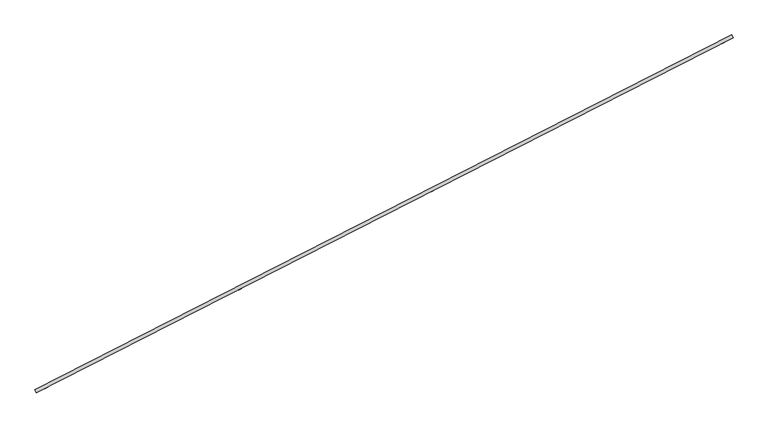
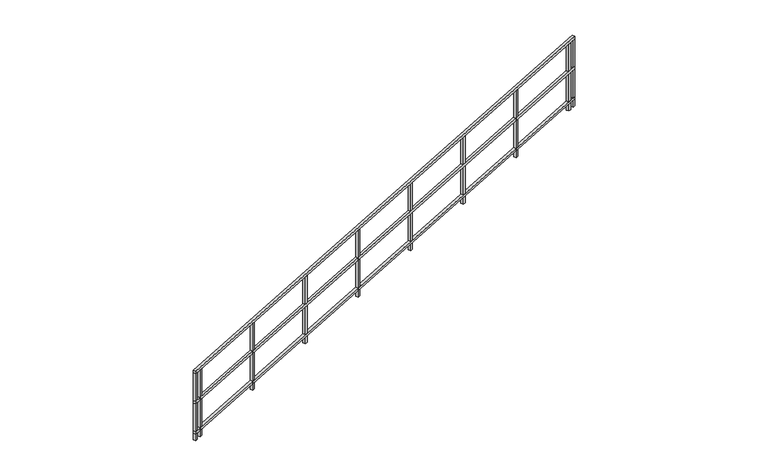
"""IFC4 building model written with IfcOpenShell, lengths in millimetres: railing geometry."""

import ifcopenshell
import ifcopenshell.guid

model = None  # the IFC model being written
_history = None  # IfcOwnerHistory: only IFC2X3 demands one
_inside = {}  # id of a spatial element -> (the spatial element, [elements in it])
_under = {}  # id of a project, library or spatial element -> (it, [spatial elements below it])
_declared = {}  # id of a project -> (the project, [libraries it declares])
_typed = {}  # id of a type object -> (the type object, [elements of that type])
_made_of = {}  # id of a material, layer set ... -> (it, [elements and type objects made of it])


def new_model(schema):
    """Start an empty IFC model of exactly this schema.

    Asked for "IFC4X3", IfcOpenShell would pick the latest addendum, in which some entities
    have other attributes; the version numbers below select the first issue.
    IFC2X3 requires an IfcOwnerHistory on every rooted entity: one is made here for all.
    """
    global model, _history
    if schema == "IFC4X3":
        model = ifcopenshell.file(schema_version=(4, 3, 0, 0))
    else:
        model = ifcopenshell.file(schema=schema)
    _inside.clear()
    _under.clear()
    _declared.clear()
    _typed.clear()
    _made_of.clear()
    _history = None
    if model.schema == "IFC2X3":
        org = make("IfcOrganization", Name="unknown")
        user = make(
            "IfcPersonAndOrganization",
            ThePerson=make("IfcPerson", FamilyName="unknown"),
            TheOrganization=org,
        )
        app = make(
            "IfcApplication",
            ApplicationDeveloper=org,
            Version="unknown",
            ApplicationFullName="unknown",
            ApplicationIdentifier="unknown",
        )
        _history = make(
            "IfcOwnerHistory",
            OwningUser=user,
            OwningApplication=app,
            ChangeAction="ADDED",
            CreationDate=0,
        )
    return model


def make(cls, **values):
    """One entity of the class cls with the attributes given. An attribute that is None is left unset."""
    return model.create_entity(
        cls, **{name: value for name, value in values.items() if value is not None}
    )


def rooted(cls, **values):
    """An entity with a GlobalId (a new one), such as an element, a storey or a relation."""
    return make(cls, GlobalId=ifcopenshell.guid.new(), OwnerHistory=_history, **values)


def si_unit(unit_type, name, prefix=None):
    """IfcSIUnit, for example si_unit("LENGTHUNIT", "METRE", prefix="MILLI")."""
    return make("IfcSIUnit", UnitType=unit_type, Prefix=prefix, Name=name)


def assignment(units):
    """IfcUnitAssignment: the units of a project."""
    return None if units is None else make("IfcUnitAssignment", Units=units)


def point(xyz):
    """IfcCartesianPoint."""
    return None if xyz is None else make("IfcCartesianPoint", Coordinates=xyz)


def direction(xyz):
    """IfcDirection."""
    return None if xyz is None else make("IfcDirection", DirectionRatios=xyz)


def frame(location, z_axis=None, x_axis=None):
    """IfcAxis2Placement3D, a coordinate frame: its origin and axes. An axis left out is left unset."""
    return make(
        "IfcAxis2Placement3D",
        Location=point(location),
        Axis=direction(z_axis),
        RefDirection=direction(x_axis),
    )


def origin():
    """The frame at (0, 0, 0) with its axes left unset."""
    return frame((0.0, 0.0, 0.0))


def place(relative_to, where):
    """IfcLocalPlacement: puts the frame where relative to a parent placement (None: the world)."""
    return make(
        "IfcLocalPlacement", PlacementRelTo=relative_to, RelativePlacement=where
    )


def context(
    kind, dimensions, precision=None, world=None, true_north=None, identifier=None
):
    """IfcGeometricRepresentationContext, for example the 3D "Model" context."""
    return make(
        "IfcGeometricRepresentationContext",
        ContextIdentifier=identifier,
        ContextType=kind,
        CoordinateSpaceDimension=dimensions,
        Precision=precision,
        WorldCoordinateSystem=world,
        TrueNorth=true_north,
    )


def project(units=None, contexts=None):
    """IfcProject with its units and contexts."""
    return rooted(
        "IfcProject",
        Name="project",
        RepresentationContexts=contexts,
        UnitsInContext=assignment(units),
    )


def spatial(cls, under=None, at=None, **own):
    """A site, building, storey or space (cls), placed at a placement, below another one or the project."""
    s = rooted(cls, ObjectPlacement=at, **own)
    if under is not None:
        _under.setdefault(under.id(), (under, []))[1].append(s)
    return s


def polyline(points):
    """IfcPolyline through the points."""
    return make("IfcPolyline", Points=[point(p) for p in points])


def outline(outer, holes=None, kind="AREA"):
    """IfcArbitraryClosedProfileDef: a profile drawn as a closed curve; with holes, ...WithVoids."""
    if holes is None:
        return make("IfcArbitraryClosedProfileDef", ProfileType=kind, OuterCurve=outer)
    return make(
        "IfcArbitraryProfileDefWithVoids",
        ProfileType=kind,
        OuterCurve=outer,
        InnerCurves=holes,
    )


def extrude(swept, where, along, depth):
    """IfcExtrudedAreaSolid: the profile swept, set in the frame where, extruded along a direction by depth."""
    return make(
        "IfcExtrudedAreaSolid",
        SweptArea=swept,
        Position=where,
        ExtrudedDirection=direction(along),
        Depth=depth,
    )


def shape(context_of_items, identifier, shape_type, items):
    """IfcShapeRepresentation: the items that make up one representation, for example the "Body"."""
    return make(
        "IfcShapeRepresentation",
        ContextOfItems=context_of_items,
        RepresentationIdentifier=identifier,
        RepresentationType=shape_type,
        Items=items,
    )


def source(mapping_origin, context_of_items, identifier, shape_type, items):
    """IfcRepresentationMap: a shape defined once, which mapped items show again and again."""
    return make(
        "IfcRepresentationMap",
        MappingOrigin=mapping_origin,
        MappedRepresentation=shape(context_of_items, identifier, shape_type, items),
    )


def transform(
    local_origin,
    x_axis=None,
    y_axis=None,
    z_axis=None,
    scale=None,
    scale2=None,
    scale3=None,
    uniform=True,
):
    """IfcCartesianTransformationOperator3D, or its non-uniform kind. x_axis, y_axis, z_axis: its Axis1, 2, 3."""
    if uniform:
        return make(
            "IfcCartesianTransformationOperator3D",
            Axis1=direction(x_axis),
            Axis2=direction(y_axis),
            LocalOrigin=point(local_origin),
            Scale=scale,
            Axis3=direction(z_axis),
        )
    return make(
        "IfcCartesianTransformationOperator3DnonUniform",
        Axis1=direction(x_axis),
        Axis2=direction(y_axis),
        LocalOrigin=point(local_origin),
        Scale=scale,
        Axis3=direction(z_axis),
        Scale2=scale2,
        Scale3=scale3,
    )


def mapped(mapping_source, mapping_target):
    """IfcMappedItem: shows the shape of a source again, moved by a transform."""
    return make(
        "IfcMappedItem", MappingSource=mapping_source, MappingTarget=mapping_target
    )


def made_of(thing, what):
    """Note that an element or type object is made of a material, layer set ...; save() writes the relation."""
    if what is not None:
        _made_of.setdefault(what.id(), (what, []))[1].append(thing)
    return thing


def element(
    cls,
    number,
    at=None,
    inside=None,
    cuts=None,
    type_object=None,
    material=None,
    context=None,
    identifier="Body",
    shape_type=None,
    held_by="IfcProductDefinitionShape",
    body=None,
    shapes=None,
    **own,
):
    """One element of the class cls, such as IfcWall. Its Tag is "e" and its number.

    at: its placement. inside: the storey or other place that contains it. cuts: it is an
    opening in that element (IfcRelVoidsElement). A single representation is given by context,
    identifier, shape_type and body (its items); several are given by shapes. held_by: the class
    of the entity that holds the representations. save() writes the other relations.
    """
    e = rooted(cls, Tag="e%d" % number, ObjectPlacement=at, **own)
    if body is not None:
        shapes = [shape(context, identifier, shape_type, body)]
    if shapes is not None:
        e.Representation = make(held_by, Representations=shapes)
    if inside is not None:
        _inside.setdefault(inside.id(), (inside, []))[1].append(e)
    if cuts is not None:
        rooted(
            "IfcRelVoidsElement", RelatingBuildingElement=cuts, RelatedOpeningElement=e
        )
    if type_object is not None:
        _typed.setdefault(type_object.id(), (type_object, []))[1].append(e)
    return made_of(e, material)


def aggregate(whole, parts):
    """IfcRelAggregates: a whole, such as a stair, and the parts it consists of."""
    return rooted("IfcRelAggregates", RelatingObject=whole, RelatedObjects=parts)


def save(model, path):
    """Write the relations noted so far, then the file.

    IfcRelAggregates (storeys below a building ...), IfcRelContainedInSpatialStructure (elements
    in a storey), IfcRelDefinesByType, IfcRelAssociatesMaterial and IfcRelDeclares: one each for
    every whole, place, type object, material and project.
    """
    for whole, parts in _under.values():
        aggregate(whole, parts)
    for where, things in _inside.values():
        rooted(
            "IfcRelContainedInSpatialStructure",
            RelatedElements=things,
            RelatingStructure=where,
        )
    for kind, things in _typed.values():
        rooted("IfcRelDefinesByType", RelatedObjects=things, RelatingType=kind)
    for what, things in _made_of.values():
        rooted("IfcRelAssociatesMaterial", RelatedObjects=things, RelatingMaterial=what)
    for by, libraries in _declared.values():
        rooted("IfcRelDeclares", RelatingContext=by, RelatedDefinitions=libraries)
    model.write(path)


def railing_8f82b1fa(model_context):
    return source(origin(), model_context, "Body", "SweptSolid", [
        extrude(outline(polyline([(54203.6748483, 45637.5924682), (54220.9718863, 45603.6451197), (46399.2676625, 41618.2877592), (46381.9706245, 41652.2351078), (54203.6748483, 45637.5924682)])), frame((0.0, 0.0, 266339.5064882), z_axis=(0.0, 0.0, 1.0), x_axis=(1.0, 0.0, 0.0)), (0.0, 0.0, 1.0), 38.1),
        extrude(outline(polyline([(54203.6748483, 45637.5924682), (54220.9718863, 45603.6451197), (46399.2676625, 41618.2877592), (46381.9706245, 41652.2351078), (54203.6748483, 45637.5924682)])), frame((0.0, 0.0, 265875.9564882), z_axis=(0.0, 0.0, 1.0), x_axis=(1.0, 0.0, 0.0)), (0.0, 0.0, 1.0), 38.1),
        extrude(outline(polyline([(54203.6748483, 45637.5924682), (54220.9718863, 45603.6451197), (46399.2676625, 41618.2877592), (46381.9706245, 41652.2351078), (54203.6748483, 45637.5924682)])), frame((0.0, 0.0, 265412.4064882), z_axis=(0.0, 0.0, 1.0), x_axis=(1.0, 0.0, 0.0)), (0.0, 0.0, 1.0), 38.1),
        extrude(outline(polyline([(46524.9904087, 41682.346698), (46491.0430601, 41665.0496599), (46473.7460221, 41698.9970085), (46507.6933706, 41716.2940465), (46524.9904087, 41682.346698)])), frame((0.0, 0.0, 265310.8064882), z_axis=(0.0, 0.0, 1.0), x_axis=(1.0, 0.0, 0.0)), (0.0, 0.0, 1.0), 1028.7),
        extrude(outline(polyline([(47611.305563, 42235.8519153), (47577.3582144, 42218.5548772), (47560.0611764, 42252.5022258), (47594.0085249, 42269.7992638), (47611.305563, 42235.8519153)])), frame((0.0, 0.0, 265310.8064882), z_axis=(0.0, 0.0, 1.0), x_axis=(1.0, 0.0, 0.0)), (0.0, 0.0, 1.0), 1028.7),
        extrude(outline(polyline([(48697.6207173, 42789.3571325), (48663.6733687, 42772.0600945), (48646.3763307, 42806.0074431), (48680.3236792, 42823.3044811), (48697.6207173, 42789.3571325)])), frame((0.0, 0.0, 265310.8064882), z_axis=(0.0, 0.0, 1.0), x_axis=(1.0, 0.0, 0.0)), (0.0, 0.0, 1.0), 1028.7),
        extrude(outline(polyline([(49783.9358716, 43342.8623498), (49749.988523, 43325.5653118), (49732.6914849, 43359.5126604), (49766.6388335, 43376.8096984), (49783.9358716, 43342.8623498)])), frame((0.0, 0.0, 265310.8064882), z_axis=(0.0, 0.0, 1.0), x_axis=(1.0, 0.0, 0.0)), (0.0, 0.0, 1.0), 1028.7),
        extrude(outline(polyline([(50870.2510258, 43896.3675671), (50836.3036773, 43879.0705291), (50819.0066392, 43913.0178776), (50852.9539878, 43930.3149157), (50870.2510258, 43896.3675671)])), frame((0.0, 0.0, 265310.8064882), z_axis=(0.0, 0.0, 1.0), x_axis=(1.0, 0.0, 0.0)), (0.0, 0.0, 1.0), 1028.7),
        extrude(outline(polyline([(51956.5661801, 44449.8727844), (51922.6188316, 44432.5757463), (51905.3217935, 44466.5230949), (51939.2691421, 44483.820133), (51956.5661801, 44449.8727844)])), frame((0.0, 0.0, 265310.8064882), z_axis=(0.0, 0.0, 1.0), x_axis=(1.0, 0.0, 0.0)), (0.0, 0.0, 1.0), 1028.7),
        extrude(outline(polyline([(53042.8813344, 45003.3780017), (53008.9339859, 44986.0809636), (52991.6369478, 45020.0283122), (53025.5842964, 45037.3253502), (53042.8813344, 45003.3780017)])), frame((0.0, 0.0, 265310.8064882), z_axis=(0.0, 0.0, 1.0), x_axis=(1.0, 0.0, 0.0)), (0.0, 0.0, 1.0), 1028.7),
        extrude(outline(polyline([(54129.1964887, 45556.883219), (54095.2491401, 45539.5861809), (54077.9521021, 45573.5335295), (54111.8994507, 45590.8305675), (54129.1964887, 45556.883219)])), frame((0.0, 0.0, 265310.8064882), z_axis=(0.0, 0.0, 1.0), x_axis=(1.0, 0.0, 0.0)), (0.0, 0.0, 1.0), 1028.7),
        extrude(outline(polyline([(46433.2150111, 41635.5847973), (46399.2676625, 41618.2877592), (46381.9706245, 41652.2351078), (46415.9179731, 41669.5321458), (46433.2150111, 41635.5847973)])), frame((0.0, 0.0, 265310.8064882), z_axis=(0.0, 0.0, 1.0), x_axis=(1.0, 0.0, 0.0)), (0.0, 0.0, 1.0), 1028.7),
        extrude(outline(polyline([(54220.9718863, 45603.6451197), (54187.0245377, 45586.3480816), (54169.7274997, 45620.2954302), (54203.6748483, 45637.5924682), (54220.9718863, 45603.6451197)])), frame((0.0, 0.0, 265310.8064882), z_axis=(0.0, 0.0, 1.0), x_axis=(1.0, 0.0, 0.0)), (0.0, 0.0, 1.0), 1028.7),
    ])


if __name__ == "__main__":
    model = new_model("IFC4")
    model_context = context("Model", 3, world=origin())
    ifc_project = project(units=[si_unit("LENGTHUNIT", "METRE", prefix="MILLI")], contexts=[model_context])
    site = spatial("IfcSite", under=ifc_project)
    building = spatial("IfcBuilding", under=site)
    placement = place(None, origin())
    railing_shape = railing_8f82b1fa(model_context)
    element("IfcRailing", 1, at=placement, inside=building, context=model_context, shape_type="MappedRepresentation", body=[
        mapped(railing_shape, transform((0.0, 0.0, 0.0), x_axis=(1.0, 0.0, 0.0), y_axis=(0.0, 1.0, 0.0), z_axis=(0.0, 0.0, 1.0))),
    ])
    save(model, "model.ifc")

# Revit data of these elements
# Element 1 (IfcRailing)
#   Materials on its faces: "Laypere Stair - Powder Coated Steel - Color as Specified"
# Materials
#   "Laypere Stair - Powder Coated Steel - Color as Specified": class "Miscellaneous", colour RGB 178 35 35, transparency 0, Keynote = "05 52 00", Model = "Powder Coated Steel - Color as Specified", Manufacturer = "LAPEYRE STAIR, INC.", Description = "Powder Coated Steel - Color as Specified", Cost = 0
